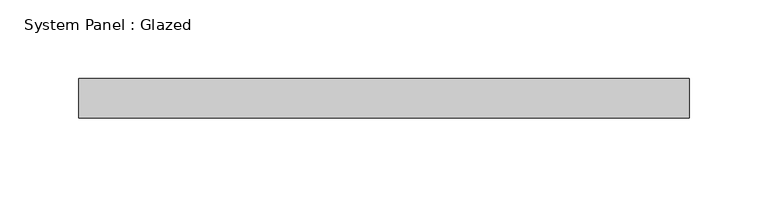
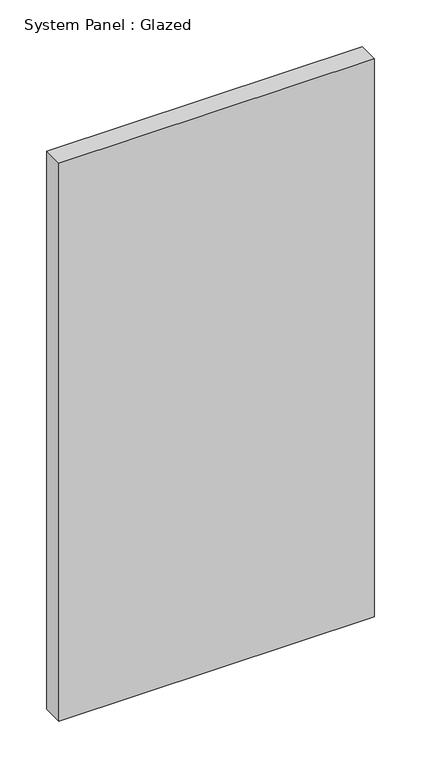
"""IFC4 building model written with IfcOpenShell, lengths in millimetres: plate geometry, System Panel : Glazed."""

from ifc_helpers import new_model, si_unit, origin, origin_with_axes, place, context, project, spatial, polyline, outline, extrude, source, transform, mapped, element, save


def system_panel_glazed_6b3d1054(model_context):
    return source(origin(), model_context, "Body", "SweptSolid", [
        extrude(outline(polyline([(193.75, 24.5), (-193.75, 24.5), (-193.75, 49.5), (193.75, 49.5), (193.75, 24.5)])), origin_with_axes(), (0.0, 0.0, 1.0), 725.0),
    ])


if __name__ == "__main__":
    model = new_model("IFC4")
    model_context = context("Model", 3, world=origin())
    ifc_project = project(units=[si_unit("LENGTHUNIT", "METRE", prefix="MILLI")], contexts=[model_context])
    site = spatial("IfcSite", under=ifc_project)
    building = spatial("IfcBuilding", under=site)
    placement = place(None, origin())
    system_panel_glazed_shape = system_panel_glazed_6b3d1054(model_context)
    element("IfcPlate", 1, ObjectType="System Panel : Glazed", at=placement, inside=building, context=model_context, shape_type="MappedRepresentation", body=[
        mapped(system_panel_glazed_shape, transform((0.0, 0.0, 0.0), x_axis=(1.0, 0.0, 0.0), y_axis=(0.0, 1.0, 0.0), z_axis=(0.0, 0.0, 1.0))),
    ])
    save(model, "model.ifc")

# Revit data of these elements
# Type "System Panel : Glazed"
#   Construction Type Id = "GSP4R"
#   Analytic Construction = "1/8 in Pilkington single glazing"
#   Visual Light Transmittance = 0.9
#   Solar Heat Gain Coefficient = 0.86
#   Heat Transfer Coefficient (U) = 6.7069 W/(m²·K)
#   Define Thermal Properties by = 1
# Element 1 (IfcPlate, "System Panel : Glazed")
#   Materials on its faces: "Glass"
# Materials
#   "Glass": class "Glass", colour RGB 0 128 192, transparency 0.9, Description = "Soda Lime Glass", Cost = 0
